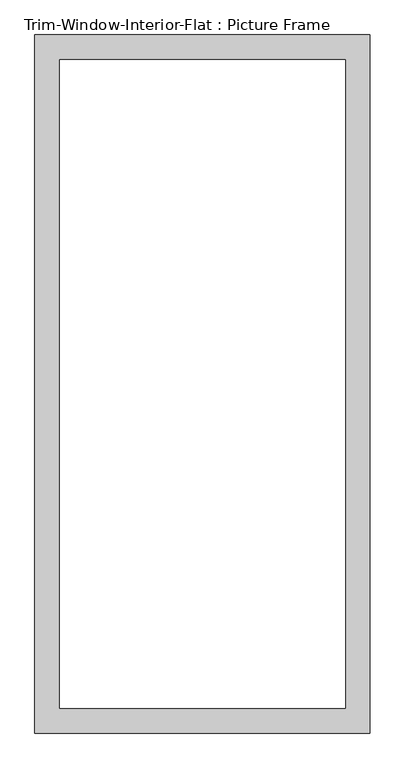
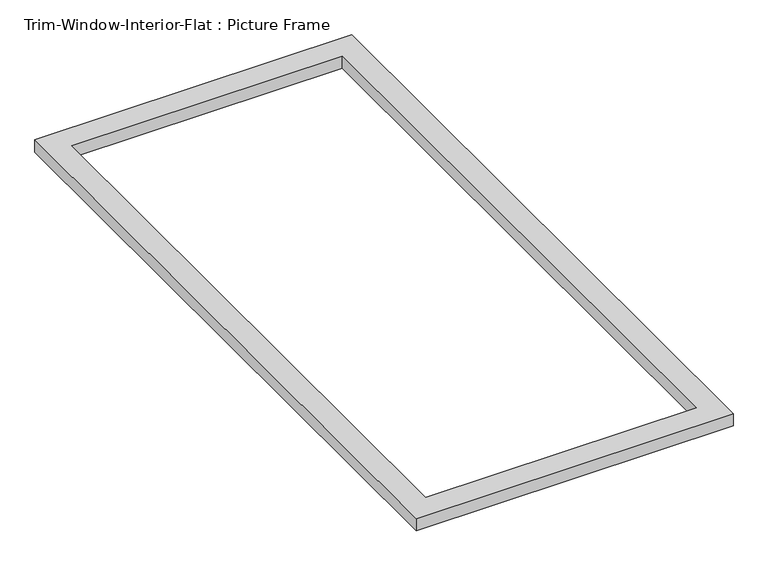
"""IFC4 building model written with IfcOpenShell, lengths in millimetres: proxy geometry, Trim-Window-Interior-Flat : Picture Frame."""

from ifc_helpers import new_model, si_unit, origin, origin_with_axes, place, context, project, spatial, polyline, outline, extrude, source, transform, mapped, element, save


def trim_window_interior_flat_picture_frame_539da632(model_context):
    return source(origin(), model_context, "Body", "SweptSolid", [
        extrude(outline(polyline([(387.35, -44.45), (-387.35, -44.45), (-387.35, 1568.45), (387.35, 1568.45), (387.35, -44.45)]), holes=[polyline([(330.2, 12.7), (330.2, 1511.3), (-330.2, 1511.3), (-330.2, 12.7), (330.2, 12.7)])]), origin_with_axes(), (0.0, 0.0, 1.0), 31.75),
    ])


if __name__ == "__main__":
    model = new_model("IFC4")
    model_context = context("Model", 3, world=origin())
    ifc_project = project(units=[si_unit("LENGTHUNIT", "METRE", prefix="MILLI")], contexts=[model_context])
    site = spatial("IfcSite", under=ifc_project)
    building = spatial("IfcBuilding", under=site)
    placement = place(None, origin())
    trim_window_interior_flat_picture_frame_shape = trim_window_interior_flat_picture_frame_539da632(model_context)
    element("IfcBuildingElementProxy", 1, Name="Trim-Window-Interior-Flat : Picture Frame", ObjectType="Trim-Window-Interior-Flat : Picture Frame", at=placement, inside=building, context=model_context, shape_type="MappedRepresentation", body=[
        mapped(trim_window_interior_flat_picture_frame_shape, transform((0.0, 0.0, 0.0), x_axis=(1.0, 0.0, 0.0), y_axis=(0.0, 1.0, 0.0), z_axis=(0.0, 0.0, 1.0))),
    ])
    save(model, "model.ifc")

# Revit data of these elements
# Type "Trim-Window-Interior-Flat : Picture Frame"
#   Trim Thickness_Picture Frame = 0' - 1 1/4"
#   Trim Width = 0' - 2 1/4"
#   Trim Thickness_with Sill = 0' - 0 3/4"
#   Sill Thickness = 0' - 1 1/4"
#   Opening Width [instance default] = 2' - 0"
#   Opening Height [instance default] = 3' - 0"
#   Default Elevation = 4' - 0"
#   Sill = no
#   Picture Frame = yes
#   Trim Material [instance default] = none
# Element 1 (IfcBuildingElementProxy, "Trim-Window-Interior-Flat : Picture Frame")
#   Opening Width = 2' - 3"
#   Opening Height = 5' - 0"
#   Trim Material = Wood - Stained
#   Materials on its faces: "Wood - Stained"
# Materials
#   "Wood - Stained": class "Wood", colour RGB 224 178 126, transparency 0, Cost = 0
